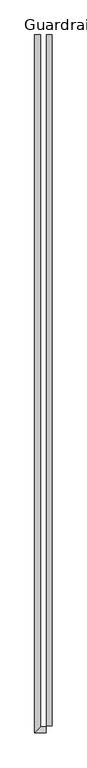
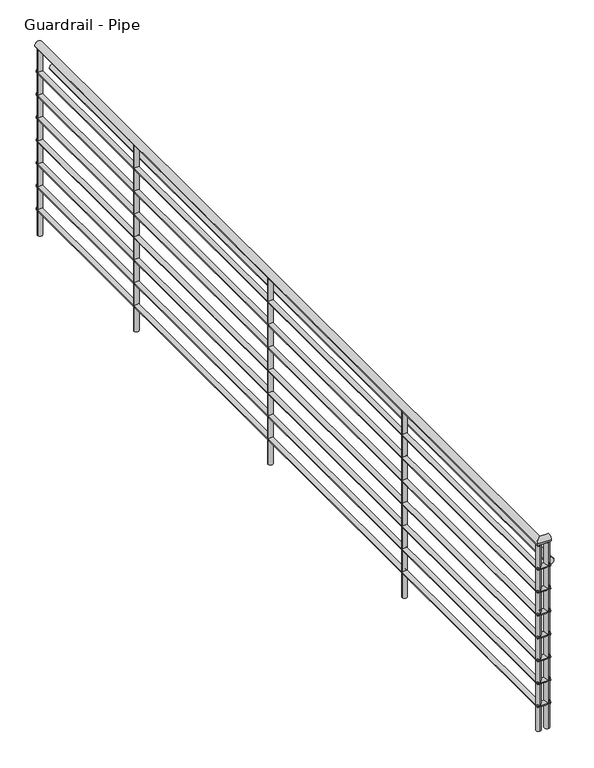
"""IFC4 building model written with IfcOpenShell, lengths in millimetres: railing geometry, Guardrail - Pipe."""

from ifc_helpers import new_model, si_unit, point, frame, frame_2d, origin, place, context, project, spatial, circle_curve, ellipse_curve, trimmed, segment, composite_curve, outline, extrude, source, transform, mapped, element, save
from ifc_brep_helpers import plane_surface, cylinder_surface, advanced_brep


def guardrail_pipe_4d6737b3(model_context):
    return source(origin(), model_context, "Body", "SolidModel", [
        advanced_brep(
        [(-10682.1293787, 596.0663228, 4705.35), (-10720.2293787, 596.0663228, 4705.35), (-10682.1293787, -3931.4836772, 4705.35), (-10720.2293787, -3969.5836772, 4705.35), (-10645.1029016, -3931.4836772, 4705.35), (-10645.1029016, -3969.5836772, 4705.35)],
        [
            (0, 1, circle_curve(frame((-10701.1793787, 596.0663228, 4705.35), z_axis=(0.0, 1.0, 0.0), x_axis=(-1.0, 0.0, 0.0)), 19.05)),
            (1, 0, circle_curve(frame((-10701.1793787, 596.0663228, 4705.35), z_axis=(0.0, 1.0, 0.0), x_axis=(-1.0, 0.0, 0.0)), 19.05)),
            (2, 3, ellipse_curve(frame((-10701.1793787, -3950.5336772, 4705.35), z_axis=(-0.7071067811865456, 0.7071067811865493, 0.0), x_axis=(-0.7071067811865492, -0.7071067811865458, 0.0)), 26.9407684, 19.05)),
            (3, 1),
            (0, 2),
            (3, 2, ellipse_curve(frame((-10701.1793787, -3950.5336772, 4705.35), z_axis=(-0.7071067811865456, 0.7071067811865493, 0.0), x_axis=(-0.7071067811865492, -0.7071067811865458, 0.0)), 26.9407684, 19.05)),
            (4, 5, circle_curve(frame((-10645.1029016, -3950.5336772, 4705.35), z_axis=(1.0, 0.0, 0.0), x_axis=(0.0, -1.0, 0.0)), 19.05)),
            (5, 4, circle_curve(frame((-10645.1029016, -3950.5336772, 4705.35), z_axis=(1.0, 0.0, 0.0), x_axis=(0.0, -1.0, 0.0)), 19.05)),
            (5, 3),
            (2, 4),
        ],
        [
            plane_surface(frame((-10701.1793787, 596.0663228, 4724.4), z_axis=(0.0, 1.0, 0.0), x_axis=(0.0, 0.0, 1.0))),
            cylinder_surface(frame((-10701.1793787, -3950.5336772, 4705.35), z_axis=(0.0, -1.0, 0.0), x_axis=(-1.0, 0.0, 0.0)), 19.05),
            plane_surface(frame((-10645.1029016, -3950.5336772, 4724.4), z_axis=(1.0, 0.0, 0.0), x_axis=(0.0, -1.0, 0.0))),
            cylinder_surface(frame((-10645.1029016, -3950.5336772, 4705.35), z_axis=(1.0, 0.0, 0.0), x_axis=(0.0, -1.0, 0.0)), 19.05),
        ],
        [
            (0, [[1, 2]]),
            (1, [[3, 4, -1, 5]]),
            (1, [[6, -5, -2, -4]]),
            (2, [[7, 8]]),
            (3, [[-8, 9, -3, 10]]),
            (3, [[-7, -10, -6, -9]]),
        ],
    ),
        advanced_brep(
        [(-10688.4793787, 596.0663228, 4559.3), (-10713.8793787, 596.0663228, 4559.3), (-10688.4793787, -3937.8336772, 4559.3), (-10713.8793787, -3963.2336772, 4559.3), (-10645.1029016, -3937.8336772, 4559.3), (-10645.1029016, -3963.2336772, 4559.3)],
        [
            (0, 1, circle_curve(frame((-10701.1793787, 596.0663228, 4559.3), z_axis=(0.0, 1.0, 0.0), x_axis=(-1.0, 0.0, 0.0)), 12.7)),
            (1, 0, circle_curve(frame((-10701.1793787, 596.0663228, 4559.3), z_axis=(0.0, 1.0, 0.0), x_axis=(-1.0, 0.0, 0.0)), 12.7)),
            (2, 3, ellipse_curve(frame((-10701.1793787, -3950.5336772, 4559.3), z_axis=(-0.7071067811865456, 0.7071067811865493, 0.0), x_axis=(-0.7071067811865492, -0.7071067811865458, 0.0)), 17.9605122, 12.7)),
            (3, 1),
            (0, 2),
            (3, 2, ellipse_curve(frame((-10701.1793787, -3950.5336772, 4559.3), z_axis=(-0.7071067811865456, 0.7071067811865493, 0.0), x_axis=(-0.7071067811865492, -0.7071067811865458, 0.0)), 17.9605122, 12.7)),
            (4, 5, circle_curve(frame((-10645.1029016, -3950.5336772, 4559.3), z_axis=(1.0, 0.0, 0.0), x_axis=(0.0, -1.0, 0.0)), 12.7)),
            (5, 4, circle_curve(frame((-10645.1029016, -3950.5336772, 4559.3), z_axis=(1.0, 0.0, 0.0), x_axis=(0.0, -1.0, 0.0)), 12.7)),
            (4, 2),
            (3, 5),
        ],
        [
            plane_surface(frame((-10701.1793787, 596.0663228, 4572.0), z_axis=(0.0, 1.0, 0.0), x_axis=(0.0, 0.0, 1.0))),
            cylinder_surface(frame((-10701.1793787, -3950.5336772, 4559.3), z_axis=(0.0, -1.0, 0.0), x_axis=(-1.0, 0.0, 0.0)), 12.7),
            plane_surface(frame((-10645.1029016, -3950.5336772, 4572.0), z_axis=(1.0, 0.0, 0.0), x_axis=(0.0, -1.0, 0.0))),
            cylinder_surface(frame((-10645.1029016, -3950.5336772, 4559.3), z_axis=(1.0, 0.0, 0.0), x_axis=(0.0, -1.0, 0.0)), 12.7),
        ],
        [
            (0, [[1, 2]]),
            (1, [[3, 4, -1, 5]]),
            (1, [[6, -5, -2, -4]]),
            (2, [[7, 8]]),
            (3, [[-7, 9, -6, 10]]),
            (3, [[-8, -10, -3, -9]]),
        ],
    ),
        advanced_brep(
        [(-10605.9293787, -3925.1336772, 4552.95), (-10644.0293787, -3925.1336772, 4552.95), (-10605.9293787, 596.0663228, 4552.95), (-10644.0293787, 596.0663228, 4552.95)],
        [
            (0, 1, circle_curve(frame((-10624.9793787, -3925.1336772, 4552.95), z_axis=(0.0, -1.0, 0.0), x_axis=(-1.0, 0.0, 0.0)), 19.05)),
            (1, 0, circle_curve(frame((-10624.9793787, -3925.1336772, 4552.95), z_axis=(0.0, -1.0, 0.0), x_axis=(-1.0, 0.0, 0.0)), 19.05)),
            (2, 3, circle_curve(frame((-10624.9793787, 596.0663228, 4552.95), z_axis=(0.0, 1.0, 0.0), x_axis=(-1.0, 0.0, 0.0)), 19.05)),
            (3, 2, circle_curve(frame((-10624.9793787, 596.0663228, 4552.95), z_axis=(0.0, 1.0, 0.0), x_axis=(-1.0, 0.0, 0.0)), 19.05)),
            (1, 3),
            (2, 0),
        ],
        [
            plane_surface(frame((-10624.9793787, -3925.1336772, 4572.0), z_axis=(0.0, -1.0, 0.0), x_axis=(0.0, 0.0, 1.0))),
            plane_surface(frame((-10624.9793787, 596.0663228, 4572.0), z_axis=(0.0, 1.0, 0.0), x_axis=(0.0, 0.0, 1.0))),
            cylinder_surface(frame((-10624.9793787, -3925.1336772, 4552.95), z_axis=(0.0, -1.0, 0.0), x_axis=(-1.0, 0.0, 0.0)), 19.05),
        ],
        [
            (0, [[1, 2]]),
            (1, [[3, 4]]),
            (2, [[-2, 5, -3, 6]]),
            (2, [[-1, -6, -4, -5]]),
        ],
    ),
        advanced_brep(
        [(-10688.4793787, 596.0663228, 4432.3), (-10713.8793787, 596.0663228, 4432.3), (-10688.4793787, -3937.8336772, 4432.3), (-10713.8793787, -3963.2336772, 4432.3), (-10645.1029016, -3937.8336772, 4432.3), (-10645.1029016, -3963.2336772, 4432.3)],
        [
            (0, 1, circle_curve(frame((-10701.1793787, 596.0663228, 4432.3), z_axis=(0.0, 1.0, 0.0), x_axis=(-1.0, 0.0, 0.0)), 12.7)),
            (1, 0, circle_curve(frame((-10701.1793787, 596.0663228, 4432.3), z_axis=(0.0, 1.0, 0.0), x_axis=(-1.0, 0.0, 0.0)), 12.7)),
            (2, 3, ellipse_curve(frame((-10701.1793787, -3950.5336772, 4432.3), z_axis=(-0.7071067811865456, 0.7071067811865493, 0.0), x_axis=(-0.7071067811865492, -0.7071067811865458, 0.0)), 17.9605122, 12.7)),
            (3, 1),
            (0, 2),
            (3, 2, ellipse_curve(frame((-10701.1793787, -3950.5336772, 4432.3), z_axis=(-0.7071067811865456, 0.7071067811865493, 0.0), x_axis=(-0.7071067811865492, -0.7071067811865458, 0.0)), 17.9605122, 12.7)),
            (4, 5, circle_curve(frame((-10645.1029016, -3950.5336772, 4432.3), z_axis=(1.0, 0.0, 0.0), x_axis=(0.0, -1.0, 0.0)), 12.7)),
            (5, 4, circle_curve(frame((-10645.1029016, -3950.5336772, 4432.3), z_axis=(1.0, 0.0, 0.0), x_axis=(0.0, -1.0, 0.0)), 12.7)),
            (4, 2),
            (3, 5),
        ],
        [
            plane_surface(frame((-10701.1793787, 596.0663228, 4445.0), z_axis=(0.0, 1.0, 0.0), x_axis=(0.0, 0.0, 1.0))),
            cylinder_surface(frame((-10701.1793787, -3950.5336772, 4432.3), z_axis=(0.0, -1.0, 0.0), x_axis=(-1.0, 0.0, 0.0)), 12.7),
            plane_surface(frame((-10645.1029016, -3950.5336772, 4445.0), z_axis=(1.0, 0.0, 0.0), x_axis=(0.0, -1.0, 0.0))),
            cylinder_surface(frame((-10645.1029016, -3950.5336772, 4432.3), z_axis=(1.0, 0.0, 0.0), x_axis=(0.0, -1.0, 0.0)), 12.7),
        ],
        [
            (0, [[1, 2]]),
            (1, [[3, 4, -1, 5]]),
            (1, [[6, -5, -2, -4]]),
            (2, [[7, 8]]),
            (3, [[-7, 9, -6, 10]]),
            (3, [[-8, -10, -3, -9]]),
        ],
    ),
        advanced_brep(
        [(-10688.4793787, 596.0663228, 4305.3), (-10713.8793787, 596.0663228, 4305.3), (-10688.4793787, -3937.8336772, 4305.3), (-10713.8793787, -3963.2336772, 4305.3), (-10645.1029016, -3937.8336772, 4305.3), (-10645.1029016, -3963.2336772, 4305.3)],
        [
            (0, 1, circle_curve(frame((-10701.1793787, 596.0663228, 4305.3), z_axis=(0.0, 1.0, 0.0), x_axis=(-1.0, 0.0, 0.0)), 12.7)),
            (1, 0, circle_curve(frame((-10701.1793787, 596.0663228, 4305.3), z_axis=(0.0, 1.0, 0.0), x_axis=(-1.0, 0.0, 0.0)), 12.7)),
            (2, 3, ellipse_curve(frame((-10701.1793787, -3950.5336772, 4305.3), z_axis=(-0.7071067811865456, 0.7071067811865493, 0.0), x_axis=(-0.7071067811865492, -0.7071067811865458, 0.0)), 17.9605122, 12.7)),
            (3, 1),
            (0, 2),
            (3, 2, ellipse_curve(frame((-10701.1793787, -3950.5336772, 4305.3), z_axis=(-0.7071067811865456, 0.7071067811865493, 0.0), x_axis=(-0.7071067811865492, -0.7071067811865458, 0.0)), 17.9605122, 12.7)),
            (4, 5, circle_curve(frame((-10645.1029016, -3950.5336772, 4305.3), z_axis=(1.0, 0.0, 0.0), x_axis=(0.0, -1.0, 0.0)), 12.7)),
            (5, 4, circle_curve(frame((-10645.1029016, -3950.5336772, 4305.3), z_axis=(1.0, 0.0, 0.0), x_axis=(0.0, -1.0, 0.0)), 12.7)),
            (4, 2),
            (3, 5),
        ],
        [
            plane_surface(frame((-10701.1793787, 596.0663228, 4318.0), z_axis=(0.0, 1.0, 0.0), x_axis=(0.0, 0.0, 1.0))),
            cylinder_surface(frame((-10701.1793787, -3950.5336772, 4305.3), z_axis=(0.0, -1.0, 0.0), x_axis=(-1.0, 0.0, 0.0)), 12.7),
            plane_surface(frame((-10645.1029016, -3950.5336772, 4318.0), z_axis=(1.0, 0.0, 0.0), x_axis=(0.0, -1.0, 0.0))),
            cylinder_surface(frame((-10645.1029016, -3950.5336772, 4305.3), z_axis=(1.0, 0.0, 0.0), x_axis=(0.0, -1.0, 0.0)), 12.7),
        ],
        [
            (0, [[1, 2]]),
            (1, [[3, 4, -1, 5]]),
            (1, [[6, -5, -2, -4]]),
            (2, [[7, 8]]),
            (3, [[-7, 9, -6, 10]]),
            (3, [[-8, -10, -3, -9]]),
        ],
    ),
        advanced_brep(
        [(-10688.4793787, 596.0663228, 4178.3), (-10713.8793787, 596.0663228, 4178.3), (-10688.4793787, -3937.8336772, 4178.3), (-10713.8793787, -3963.2336772, 4178.3), (-10645.1029016, -3937.8336772, 4178.3), (-10645.1029016, -3963.2336772, 4178.3)],
        [
            (0, 1, circle_curve(frame((-10701.1793787, 596.0663228, 4178.3), z_axis=(0.0, 1.0, 0.0), x_axis=(-1.0, 0.0, 0.0)), 12.7)),
            (1, 0, circle_curve(frame((-10701.1793787, 596.0663228, 4178.3), z_axis=(0.0, 1.0, 0.0), x_axis=(-1.0, 0.0, 0.0)), 12.7)),
            (2, 3, ellipse_curve(frame((-10701.1793787, -3950.5336772, 4178.3), z_axis=(-0.7071067811865456, 0.7071067811865493, 0.0), x_axis=(-0.7071067811865492, -0.7071067811865458, 0.0)), 17.9605122, 12.7)),
            (3, 1),
            (0, 2),
            (3, 2, ellipse_curve(frame((-10701.1793787, -3950.5336772, 4178.3), z_axis=(-0.7071067811865456, 0.7071067811865493, 0.0), x_axis=(-0.7071067811865492, -0.7071067811865458, 0.0)), 17.9605122, 12.7)),
            (4, 5, circle_curve(frame((-10645.1029016, -3950.5336772, 4178.3), z_axis=(1.0, 0.0, 0.0), x_axis=(0.0, -1.0, 0.0)), 12.7)),
            (5, 4, circle_curve(frame((-10645.1029016, -3950.5336772, 4178.3), z_axis=(1.0, 0.0, 0.0), x_axis=(0.0, -1.0, 0.0)), 12.7)),
            (4, 2),
            (3, 5),
        ],
        [
            plane_surface(frame((-10701.1793787, 596.0663228, 4191.0), z_axis=(0.0, 1.0, 0.0), x_axis=(0.0, 0.0, 1.0))),
            cylinder_surface(frame((-10701.1793787, -3950.5336772, 4178.3), z_axis=(0.0, -1.0, 0.0), x_axis=(-1.0, 0.0, 0.0)), 12.7),
            plane_surface(frame((-10645.1029016, -3950.5336772, 4191.0), z_axis=(1.0, 0.0, 0.0), x_axis=(0.0, -1.0, 0.0))),
            cylinder_surface(frame((-10645.1029016, -3950.5336772, 4178.3), z_axis=(1.0, 0.0, 0.0), x_axis=(0.0, -1.0, 0.0)), 12.7),
        ],
        [
            (0, [[1, 2]]),
            (1, [[3, 4, -1, 5]]),
            (1, [[6, -5, -2, -4]]),
            (2, [[7, 8]]),
            (3, [[-7, 9, -6, 10]]),
            (3, [[-8, -10, -3, -9]]),
        ],
    ),
        advanced_brep(
        [(-10688.4793787, 596.0663228, 4051.3), (-10713.8793787, 596.0663228, 4051.3), (-10688.4793787, -3937.8336772, 4051.3), (-10713.8793787, -3963.2336772, 4051.3), (-10645.1029016, -3937.8336772, 4051.3), (-10645.1029016, -3963.2336772, 4051.3)],
        [
            (0, 1, circle_curve(frame((-10701.1793787, 596.0663228, 4051.3), z_axis=(0.0, 1.0, 0.0), x_axis=(-1.0, 0.0, 0.0)), 12.7)),
            (1, 0, circle_curve(frame((-10701.1793787, 596.0663228, 4051.3), z_axis=(0.0, 1.0, 0.0), x_axis=(-1.0, 0.0, 0.0)), 12.7)),
            (2, 3, ellipse_curve(frame((-10701.1793787, -3950.5336772, 4051.3), z_axis=(-0.7071067811865456, 0.7071067811865493, 0.0), x_axis=(-0.7071067811865492, -0.7071067811865458, 0.0)), 17.9605122, 12.7)),
            (3, 1),
            (0, 2),
            (3, 2, ellipse_curve(frame((-10701.1793787, -3950.5336772, 4051.3), z_axis=(-0.7071067811865456, 0.7071067811865493, 0.0), x_axis=(-0.7071067811865492, -0.7071067811865458, 0.0)), 17.9605122, 12.7)),
            (4, 5, circle_curve(frame((-10645.1029016, -3950.5336772, 4051.3), z_axis=(1.0, 0.0, 0.0), x_axis=(0.0, -1.0, 0.0)), 12.7)),
            (5, 4, circle_curve(frame((-10645.1029016, -3950.5336772, 4051.3), z_axis=(1.0, 0.0, 0.0), x_axis=(0.0, -1.0, 0.0)), 12.7)),
            (4, 2),
            (3, 5),
        ],
        [
            plane_surface(frame((-10701.1793787, 596.0663228, 4064.0), z_axis=(0.0, 1.0, 0.0), x_axis=(0.0, 0.0, 1.0))),
            cylinder_surface(frame((-10701.1793787, -3950.5336772, 4051.3), z_axis=(0.0, -1.0, 0.0), x_axis=(-1.0, 0.0, 0.0)), 12.7),
            plane_surface(frame((-10645.1029016, -3950.5336772, 4064.0), z_axis=(1.0, 0.0, 0.0), x_axis=(0.0, -1.0, 0.0))),
            cylinder_surface(frame((-10645.1029016, -3950.5336772, 4051.3), z_axis=(1.0, 0.0, 0.0), x_axis=(0.0, -1.0, 0.0)), 12.7),
        ],
        [
            (0, [[1, 2]]),
            (1, [[3, 4, -1, 5]]),
            (1, [[6, -5, -2, -4]]),
            (2, [[7, 8]]),
            (3, [[-7, 9, -6, 10]]),
            (3, [[-8, -10, -3, -9]]),
        ],
    ),
        advanced_brep(
        [(-10688.4793787, 596.0663228, 3924.3), (-10713.8793787, 596.0663228, 3924.3), (-10688.4793787, -3937.8336772, 3924.3), (-10713.8793787, -3963.2336772, 3924.3), (-10645.1029016, -3937.8336772, 3924.3), (-10645.1029016, -3963.2336772, 3924.3)],
        [
            (0, 1, circle_curve(frame((-10701.1793787, 596.0663228, 3924.3), z_axis=(0.0, 1.0, 0.0), x_axis=(-1.0, 0.0, 0.0)), 12.7)),
            (1, 0, circle_curve(frame((-10701.1793787, 596.0663228, 3924.3), z_axis=(0.0, 1.0, 0.0), x_axis=(-1.0, 0.0, 0.0)), 12.7)),
            (2, 3, ellipse_curve(frame((-10701.1793787, -3950.5336772, 3924.3), z_axis=(-0.7071067811865456, 0.7071067811865493, 0.0), x_axis=(-0.7071067811865492, -0.7071067811865458, 0.0)), 17.9605122, 12.7)),
            (3, 1),
            (0, 2),
            (3, 2, ellipse_curve(frame((-10701.1793787, -3950.5336772, 3924.3), z_axis=(-0.7071067811865456, 0.7071067811865493, 0.0), x_axis=(-0.7071067811865492, -0.7071067811865458, 0.0)), 17.9605122, 12.7)),
            (4, 5, circle_curve(frame((-10645.1029016, -3950.5336772, 3924.3), z_axis=(1.0, 0.0, 0.0), x_axis=(0.0, -1.0, 0.0)), 12.7)),
            (5, 4, circle_curve(frame((-10645.1029016, -3950.5336772, 3924.3), z_axis=(1.0, 0.0, 0.0), x_axis=(0.0, -1.0, 0.0)), 12.7)),
            (4, 2),
            (3, 5),
        ],
        [
            plane_surface(frame((-10701.1793787, 596.0663228, 3937.0), z_axis=(0.0, 1.0, 0.0), x_axis=(0.0, 0.0, 1.0))),
            cylinder_surface(frame((-10701.1793787, -3950.5336772, 3924.3), z_axis=(0.0, -1.0, 0.0), x_axis=(-1.0, 0.0, 0.0)), 12.7),
            plane_surface(frame((-10645.1029016, -3950.5336772, 3937.0), z_axis=(1.0, 0.0, 0.0), x_axis=(0.0, -1.0, 0.0))),
            cylinder_surface(frame((-10645.1029016, -3950.5336772, 3924.3), z_axis=(1.0, 0.0, 0.0), x_axis=(0.0, -1.0, 0.0)), 12.7),
        ],
        [
            (0, [[1, 2]]),
            (1, [[3, 4, -1, 5]]),
            (1, [[6, -5, -2, -4]]),
            (2, [[7, 8]]),
            (3, [[-7, 9, -6, 10]]),
            (3, [[-8, -10, -3, -9]]),
        ],
    ),
        advanced_brep(
        [(-10688.4793787, 596.0663228, 3797.3), (-10713.8793787, 596.0663228, 3797.3), (-10688.4793787, -3937.8336772, 3797.3), (-10713.8793787, -3963.2336772, 3797.3), (-10645.1029016, -3937.8336772, 3797.3), (-10645.1029016, -3963.2336772, 3797.3)],
        [
            (0, 1, circle_curve(frame((-10701.1793787, 596.0663228, 3797.3), z_axis=(0.0, 1.0, 0.0), x_axis=(-1.0, 0.0, 0.0)), 12.7)),
            (1, 0, circle_curve(frame((-10701.1793787, 596.0663228, 3797.3), z_axis=(0.0, 1.0, 0.0), x_axis=(-1.0, 0.0, 0.0)), 12.7)),
            (2, 3, ellipse_curve(frame((-10701.1793787, -3950.5336772, 3797.3), z_axis=(-0.7071067811865456, 0.7071067811865493, 0.0), x_axis=(-0.7071067811865492, -0.7071067811865458, 0.0)), 17.9605122, 12.7)),
            (3, 1),
            (0, 2),
            (3, 2, ellipse_curve(frame((-10701.1793787, -3950.5336772, 3797.3), z_axis=(-0.7071067811865456, 0.7071067811865493, 0.0), x_axis=(-0.7071067811865492, -0.7071067811865458, 0.0)), 17.9605122, 12.7)),
            (4, 5, circle_curve(frame((-10645.1029016, -3950.5336772, 3797.3), z_axis=(1.0, 0.0, 0.0), x_axis=(0.0, -1.0, 0.0)), 12.7)),
            (5, 4, circle_curve(frame((-10645.1029016, -3950.5336772, 3797.3), z_axis=(1.0, 0.0, 0.0), x_axis=(0.0, -1.0, 0.0)), 12.7)),
            (4, 2),
            (3, 5),
        ],
        [
            plane_surface(frame((-10701.1793787, 596.0663228, 3810.0), z_axis=(0.0, 1.0, 0.0), x_axis=(0.0, 0.0, 1.0))),
            cylinder_surface(frame((-10701.1793787, -3950.5336772, 3797.3), z_axis=(0.0, -1.0, 0.0), x_axis=(-1.0, 0.0, 0.0)), 12.7),
            plane_surface(frame((-10645.1029016, -3950.5336772, 3810.0), z_axis=(1.0, 0.0, 0.0), x_axis=(0.0, -1.0, 0.0))),
            cylinder_surface(frame((-10645.1029016, -3950.5336772, 3797.3), z_axis=(1.0, 0.0, 0.0), x_axis=(0.0, -1.0, 0.0)), 12.7),
        ],
        [
            (0, [[1, 2]]),
            (1, [[3, 4, -1, 5]]),
            (1, [[6, -5, -2, -4]]),
            (2, [[7, 8]]),
            (3, [[-7, 9, -6, 10]]),
            (3, [[-8, -10, -3, -9]]),
        ],
    ),
        extrude(outline(composite_curve([segment(trimmed(circle_curve(frame_2d((-10701.1793787, -292.9336772)), 12.7), [point((-10688.4793787, -292.9336772))], [point((-10713.8793787, -292.9336772))], False, "CARTESIAN"), True, "CONTINUOUS"), segment(trimmed(circle_curve(frame_2d((-10701.1793787, -292.9336772)), 12.7), [point((-10713.8793787, -292.9336772))], [point((-10688.4793787, -292.9336772))], False, "CARTESIAN"), True, "CONTINUOUS")], self_intersect=False)), frame((0.0, 0.0, 3657.6), z_axis=(0.0, 0.0, 1.0), x_axis=(1.0, 0.0, 0.0)), (0.0, 0.0, 1.0), 1028.7),
        extrude(outline(composite_curve([segment(trimmed(circle_curve(frame_2d((-10701.1793787, -1512.1336772)), 12.7), [point((-10688.4793787, -1512.1336772))], [point((-10713.8793787, -1512.1336772))], False, "CARTESIAN"), True, "CONTINUOUS"), segment(trimmed(circle_curve(frame_2d((-10701.1793787, -1512.1336772)), 12.7), [point((-10713.8793787, -1512.1336772))], [point((-10688.4793787, -1512.1336772))], False, "CARTESIAN"), True, "CONTINUOUS")], self_intersect=False)), frame((0.0, 0.0, 3657.6), z_axis=(0.0, 0.0, 1.0), x_axis=(1.0, 0.0, 0.0)), (0.0, 0.0, 1.0), 1028.7),
        extrude(outline(composite_curve([segment(trimmed(circle_curve(frame_2d((-10701.1793787, -2731.3336772)), 12.7), [point((-10688.4793787, -2731.3336772))], [point((-10713.8793787, -2731.3336772))], False, "CARTESIAN"), True, "CONTINUOUS"), segment(trimmed(circle_curve(frame_2d((-10701.1793787, -2731.3336772)), 12.7), [point((-10713.8793787, -2731.3336772))], [point((-10688.4793787, -2731.3336772))], False, "CARTESIAN"), True, "CONTINUOUS")], self_intersect=False)), frame((0.0, 0.0, 3657.6), z_axis=(0.0, 0.0, 1.0), x_axis=(1.0, 0.0, 0.0)), (0.0, 0.0, 1.0), 1028.7),
        extrude(outline(composite_curve([segment(trimmed(circle_curve(frame_2d((-10701.1793787, -3950.5336772)), 12.7), [point((-10701.1793787, -3937.8336772))], [point((-10701.1793787, -3963.2336772))], False, "CARTESIAN"), True, "CONTINUOUS"), segment(trimmed(circle_curve(frame_2d((-10701.1793787, -3950.5336772)), 12.7), [point((-10701.1793787, -3963.2336772))], [point((-10701.1793787, -3937.8336772))], False, "CARTESIAN"), True, "CONTINUOUS")], self_intersect=False)), frame((0.0, 0.0, 3657.6), z_axis=(0.0, 0.0, 1.0), x_axis=(1.0, 0.0, 0.0)), (0.0, 0.0, 1.0), 1028.7),
        extrude(outline(composite_curve([segment(trimmed(circle_curve(frame_2d((-10701.1793787, 583.3663228)), 12.7), [point((-10688.4793787, 583.3663228))], [point((-10713.8793787, 583.3663228))], False, "CARTESIAN"), True, "CONTINUOUS"), segment(trimmed(circle_curve(frame_2d((-10701.1793787, 583.3663228)), 12.7), [point((-10713.8793787, 583.3663228))], [point((-10688.4793787, 583.3663228))], False, "CARTESIAN"), True, "CONTINUOUS")], self_intersect=False)), frame((0.0, 0.0, 3657.6), z_axis=(0.0, 0.0, 1.0), x_axis=(1.0, 0.0, 0.0)), (0.0, 0.0, 1.0), 1028.7),
        extrude(outline(composite_curve([segment(trimmed(circle_curve(frame_2d((-10657.8029016, -3950.5336772)), 12.7), [point((-10657.8029016, -3937.8336772))], [point((-10657.8029016, -3963.2336772))], False, "CARTESIAN"), True, "CONTINUOUS"), segment(trimmed(circle_curve(frame_2d((-10657.8029016, -3950.5336772)), 12.7), [point((-10657.8029016, -3963.2336772))], [point((-10657.8029016, -3937.8336772))], False, "CARTESIAN"), True, "CONTINUOUS")], self_intersect=False)), frame((0.0, 0.0, 3657.6), z_axis=(0.0, 0.0, 1.0), x_axis=(1.0, 0.0, 0.0)), (0.0, 0.0, 1.0), 1028.7),
    ])


if __name__ == "__main__":
    model = new_model("IFC4")
    model_context = context("Model", 3, world=origin())
    ifc_project = project(units=[si_unit("LENGTHUNIT", "METRE", prefix="MILLI")], contexts=[model_context])
    site = spatial("IfcSite", under=ifc_project)
    building = spatial("IfcBuilding", under=site)
    placement = place(None, origin())
    guardrail_pipe_shape = guardrail_pipe_4d6737b3(model_context)
    element("IfcRailing", 1, ObjectType="Guardrail - Pipe", at=placement, inside=building, context=model_context, shape_type="MappedRepresentation", body=[
        mapped(guardrail_pipe_shape, transform((0.0, 0.0, 0.0), x_axis=(1.0, 0.0, 0.0), y_axis=(0.0, 1.0, 0.0), z_axis=(0.0, 0.0, 1.0))),
    ])
    save(model, "model.ifc")

# Revit data of these elements
# Element 1 (IfcRailing, "Guardrail - Pipe")
#   Materials on its faces: "Plastic - Vinyl Cove Base"
# Materials
#   "Plastic - Vinyl Cove Base": class "Plastic", colour RGB 5 5 5, transparency 0, Cost = 0
